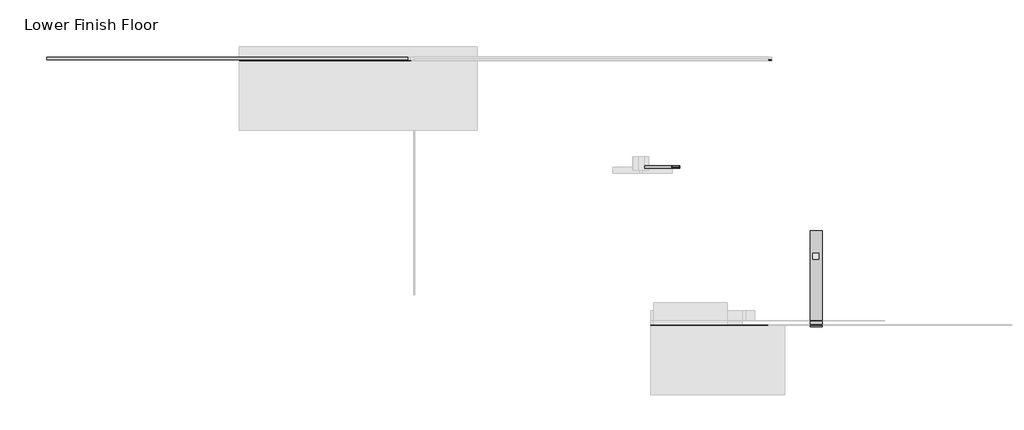
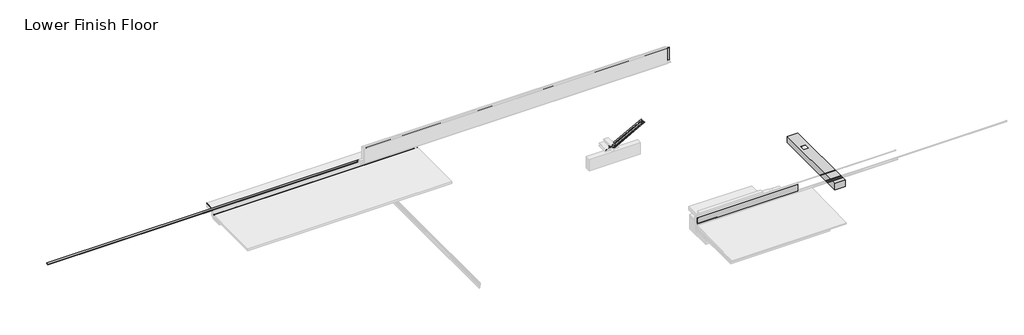
# One storey, part 1 of 2: 8 proxies, 2 beams.
"""IFC4 building model written with IfcOpenShell, lengths in millimetres."""

import ifcopenshell
import ifcopenshell.guid

model = None  # the IFC model being written
_history = None  # IfcOwnerHistory: only IFC2X3 demands one
_inside = {}  # id of a spatial element -> (the spatial element, [elements in it])
_under = {}  # id of a project, library or spatial element -> (it, [spatial elements below it])
_declared = {}  # id of a project -> (the project, [libraries it declares])
_typed = {}  # id of a type object -> (the type object, [elements of that type])
_made_of = {}  # id of a material, layer set ... -> (it, [elements and type objects made of it])


def new_model(schema):
    """Start an empty IFC model of exactly this schema.

    Asked for "IFC4X3", IfcOpenShell would pick the latest addendum, in which some entities
    have other attributes; the version numbers below select the first issue.
    IFC2X3 requires an IfcOwnerHistory on every rooted entity: one is made here for all.
    """
    global model, _history
    if schema == "IFC4X3":
        model = ifcopenshell.file(schema_version=(4, 3, 0, 0))
    else:
        model = ifcopenshell.file(schema=schema)
    _inside.clear()
    _under.clear()
    _declared.clear()
    _typed.clear()
    _made_of.clear()
    _history = None
    if model.schema == "IFC2X3":
        org = make("IfcOrganization", Name="unknown")
        user = make(
            "IfcPersonAndOrganization",
            ThePerson=make("IfcPerson", FamilyName="unknown"),
            TheOrganization=org,
        )
        app = make(
            "IfcApplication",
            ApplicationDeveloper=org,
            Version="unknown",
            ApplicationFullName="unknown",
            ApplicationIdentifier="unknown",
        )
        _history = make(
            "IfcOwnerHistory",
            OwningUser=user,
            OwningApplication=app,
            ChangeAction="ADDED",
            CreationDate=0,
        )
    return model


def make(cls, **values):
    """One entity of the class cls with the attributes given. An attribute that is None is left unset."""
    return model.create_entity(
        cls, **{name: value for name, value in values.items() if value is not None}
    )


def rooted(cls, **values):
    """An entity with a GlobalId (a new one), such as an element, a storey or a relation."""
    return make(cls, GlobalId=ifcopenshell.guid.new(), OwnerHistory=_history, **values)


def si_unit(unit_type, name, prefix=None):
    """IfcSIUnit, for example si_unit("LENGTHUNIT", "METRE", prefix="MILLI")."""
    return make("IfcSIUnit", UnitType=unit_type, Prefix=prefix, Name=name)


def assignment(units):
    """IfcUnitAssignment: the units of a project."""
    return None if units is None else make("IfcUnitAssignment", Units=units)


def point(xyz):
    """IfcCartesianPoint."""
    return None if xyz is None else make("IfcCartesianPoint", Coordinates=xyz)


def direction(xyz):
    """IfcDirection."""
    return None if xyz is None else make("IfcDirection", DirectionRatios=xyz)


def frame(location, z_axis=None, x_axis=None):
    """IfcAxis2Placement3D, a coordinate frame: its origin and axes. An axis left out is left unset."""
    return make(
        "IfcAxis2Placement3D",
        Location=point(location),
        Axis=direction(z_axis),
        RefDirection=direction(x_axis),
    )


def frame_2d(location, x_axis=None):
    """IfcAxis2Placement2D, a coordinate frame in the plane: its origin and x axis."""
    return make(
        "IfcAxis2Placement2D", Location=point(location), RefDirection=direction(x_axis)
    )


def origin():
    """The frame at (0, 0, 0) with its axes left unset."""
    return frame((0.0, 0.0, 0.0))


def place(relative_to, where):
    """IfcLocalPlacement: puts the frame where relative to a parent placement (None: the world)."""
    return make(
        "IfcLocalPlacement", PlacementRelTo=relative_to, RelativePlacement=where
    )


def context(
    kind, dimensions, precision=None, world=None, true_north=None, identifier=None
):
    """IfcGeometricRepresentationContext, for example the 3D "Model" context."""
    return make(
        "IfcGeometricRepresentationContext",
        ContextIdentifier=identifier,
        ContextType=kind,
        CoordinateSpaceDimension=dimensions,
        Precision=precision,
        WorldCoordinateSystem=world,
        TrueNorth=true_north,
    )


def project(units=None, contexts=None):
    """IfcProject with its units and contexts."""
    return rooted(
        "IfcProject",
        Name="project",
        RepresentationContexts=contexts,
        UnitsInContext=assignment(units),
    )


def spatial(cls, under=None, at=None, **own):
    """A site, building, storey or space (cls), placed at a placement, below another one or the project."""
    s = rooted(cls, ObjectPlacement=at, **own)
    if under is not None:
        _under.setdefault(under.id(), (under, []))[1].append(s)
    return s


def polyline(points):
    """IfcPolyline through the points."""
    return make("IfcPolyline", Points=[point(p) for p in points])


def circle_curve(where, radius):
    """IfcCircle in the frame where."""
    return make("IfcCircle", Position=where, Radius=radius)


def ellipse_curve(where, semi_axis1, semi_axis2):
    """IfcEllipse in the frame where."""
    return make(
        "IfcEllipse", Position=where, SemiAxis1=semi_axis1, SemiAxis2=semi_axis2
    )


def trimmed(basis, trim1, trim2, sense, master):
    """IfcTrimmedCurve: the piece of a basis curve between two trims."""
    return make(
        "IfcTrimmedCurve",
        BasisCurve=basis,
        Trim1=trim1,
        Trim2=trim2,
        SenseAgreement=sense,
        MasterRepresentation=master,
    )


def segment(curve, same_sense, transition):
    """IfcCompositeCurveSegment."""
    return make(
        "IfcCompositeCurveSegment",
        Transition=transition,
        SameSense=same_sense,
        ParentCurve=curve,
    )


def composite_curve(segments, self_intersect=None):
    """IfcCompositeCurve: segments joined end to end."""
    return make("IfcCompositeCurve", Segments=segments, SelfIntersect=self_intersect)


def outline(outer, holes=None, kind="AREA"):
    """IfcArbitraryClosedProfileDef: a profile drawn as a closed curve; with holes, ...WithVoids."""
    if holes is None:
        return make("IfcArbitraryClosedProfileDef", ProfileType=kind, OuterCurve=outer)
    return make(
        "IfcArbitraryProfileDefWithVoids",
        ProfileType=kind,
        OuterCurve=outer,
        InnerCurves=holes,
    )


def extrude(swept, where, along, depth):
    """IfcExtrudedAreaSolid: the profile swept, set in the frame where, extruded along a direction by depth."""
    return make(
        "IfcExtrudedAreaSolid",
        SweptArea=swept,
        Position=where,
        ExtrudedDirection=direction(along),
        Depth=depth,
    )


def shape(context_of_items, identifier, shape_type, items):
    """IfcShapeRepresentation: the items that make up one representation, for example the "Body"."""
    return make(
        "IfcShapeRepresentation",
        ContextOfItems=context_of_items,
        RepresentationIdentifier=identifier,
        RepresentationType=shape_type,
        Items=items,
    )


def source(mapping_origin, context_of_items, identifier, shape_type, items):
    """IfcRepresentationMap: a shape defined once, which mapped items show again and again."""
    return make(
        "IfcRepresentationMap",
        MappingOrigin=mapping_origin,
        MappedRepresentation=shape(context_of_items, identifier, shape_type, items),
    )


def transform(
    local_origin,
    x_axis=None,
    y_axis=None,
    z_axis=None,
    scale=None,
    scale2=None,
    scale3=None,
    uniform=True,
):
    """IfcCartesianTransformationOperator3D, or its non-uniform kind. x_axis, y_axis, z_axis: its Axis1, 2, 3."""
    if uniform:
        return make(
            "IfcCartesianTransformationOperator3D",
            Axis1=direction(x_axis),
            Axis2=direction(y_axis),
            LocalOrigin=point(local_origin),
            Scale=scale,
            Axis3=direction(z_axis),
        )
    return make(
        "IfcCartesianTransformationOperator3DnonUniform",
        Axis1=direction(x_axis),
        Axis2=direction(y_axis),
        LocalOrigin=point(local_origin),
        Scale=scale,
        Axis3=direction(z_axis),
        Scale2=scale2,
        Scale3=scale3,
    )


def mapped(mapping_source, mapping_target):
    """IfcMappedItem: shows the shape of a source again, moved by a transform."""
    return make(
        "IfcMappedItem", MappingSource=mapping_source, MappingTarget=mapping_target
    )


def made_of(thing, what):
    """Note that an element or type object is made of a material, layer set ...; save() writes the relation."""
    if what is not None:
        _made_of.setdefault(what.id(), (what, []))[1].append(thing)
    return thing


def element(
    cls,
    number,
    at=None,
    inside=None,
    cuts=None,
    type_object=None,
    material=None,
    context=None,
    identifier="Body",
    shape_type=None,
    held_by="IfcProductDefinitionShape",
    body=None,
    shapes=None,
    **own,
):
    """One element of the class cls, such as IfcWall. Its Tag is "e" and its number.

    at: its placement. inside: the storey or other place that contains it. cuts: it is an
    opening in that element (IfcRelVoidsElement). A single representation is given by context,
    identifier, shape_type and body (its items); several are given by shapes. held_by: the class
    of the entity that holds the representations. save() writes the other relations.
    """
    e = rooted(cls, Tag="e%d" % number, ObjectPlacement=at, **own)
    if body is not None:
        shapes = [shape(context, identifier, shape_type, body)]
    if shapes is not None:
        e.Representation = make(held_by, Representations=shapes)
    if inside is not None:
        _inside.setdefault(inside.id(), (inside, []))[1].append(e)
    if cuts is not None:
        rooted(
            "IfcRelVoidsElement", RelatingBuildingElement=cuts, RelatedOpeningElement=e
        )
    if type_object is not None:
        _typed.setdefault(type_object.id(), (type_object, []))[1].append(e)
    return made_of(e, material)


def aggregate(whole, parts):
    """IfcRelAggregates: a whole, such as a stair, and the parts it consists of."""
    return rooted("IfcRelAggregates", RelatingObject=whole, RelatedObjects=parts)


def save(model, path):
    """Write the relations noted so far, then the file.

    IfcRelAggregates (storeys below a building ...), IfcRelContainedInSpatialStructure (elements
    in a storey), IfcRelDefinesByType, IfcRelAssociatesMaterial and IfcRelDeclares: one each for
    every whole, place, type object, material and project.
    """
    for whole, parts in _under.values():
        aggregate(whole, parts)
    for where, things in _inside.values():
        rooted(
            "IfcRelContainedInSpatialStructure",
            RelatedElements=things,
            RelatingStructure=where,
        )
    for kind, things in _typed.values():
        rooted("IfcRelDefinesByType", RelatedObjects=things, RelatingType=kind)
    for what, things in _made_of.values():
        rooted("IfcRelAssociatesMaterial", RelatedObjects=things, RelatingMaterial=what)
    for by, libraries in _declared.values():
        rooted("IfcRelDeclares", RelatingContext=by, RelatedDefinitions=libraries)
    model.write(path)


def plane_surface(at):
    """IfcPlane: the flat surface through the origin of the frame at, square to its z axis."""
    return make("IfcPlane", Position=at)


def cylinder_surface(at, radius):
    """IfcCylindricalSurface: all points at the distance radius from the z axis of the frame at."""
    return make("IfcCylindricalSurface", Position=at, Radius=radius)


def revolved_surface(curve, axis_point, axis_direction):
    """IfcSurfaceOfRevolution: the curve turned about the line through axis_point along axis_direction."""
    return make(
        "IfcSurfaceOfRevolution",
        SweptCurve=make("IfcArbitraryOpenProfileDef", ProfileType="CURVE", Curve=curve),
        AxisPosition=make("IfcAxis1Placement", Location=point(axis_point), Axis=direction(axis_direction)),
    )


def advanced_brep(points, edges, surfaces, faces):
    """IfcAdvancedBrep: a solid bounded by faces that lie on surfaces and meet in shared edges.

    An edge is (start, end): straight between two places in points (the first is 0);
    or (start, end, curve); or (start, end, curve, False) where it runs against its curve.
    A face is (place in surfaces, loops), or (place, loops, False) where it looks against
    its surface's normal. A loop lists edges by number (the first is 1), with a minus sign
    where the edge is run from its end to its start. The first loop is the outer one.
    """
    corners = [point(p) for p in points]
    vertices = [make("IfcVertexPoint", VertexGeometry=c) for c in corners]
    made = []
    for start, end, *more in edges:
        made.append(
            make(
                "IfcEdgeCurve",
                EdgeStart=vertices[start],
                EdgeEnd=vertices[end],
                EdgeGeometry=more[0] if more else make("IfcPolyline", Points=[corners[start], corners[end]]),
                SameSense=more[1] if len(more) > 1 else True,
            )
        )
    hull = []
    for where, loops, *sense in faces:
        bounds = []
        for j, loop in enumerate(loops):
            ring = [make("IfcOrientedEdge", EdgeElement=made[abs(k) - 1], Orientation=k > 0) for k in loop]
            bounds.append(
                make(
                    "IfcFaceOuterBound" if j == 0 else "IfcFaceBound",
                    Bound=make("IfcEdgeLoop", EdgeList=ring),
                    Orientation=True,
                )
            )
        hull.append(make("IfcAdvancedFace", Bounds=bounds, FaceSurface=surfaces[where], SameSense=sense[0] if sense else True))
    return make("IfcAdvancedBrep", Outer=make("IfcClosedShell", CfsFaces=hull))


def w_wide_flange_w10x22_c2580360(model_context):
    return source(origin(), model_context, "Body", "SweptSolid", [
        extrude(outline(composite_curve([segment(polyline([(73.025, -120.396), (73.025, -129.54), (-73.025, -129.54), (-73.025, -120.396), (-17.7165, -120.396)]), True, "CONTINUOUS"), segment(trimmed(circle_curve(frame_2d((-17.7165, -105.7275)), 14.6685), [point((-17.7165, -120.396))], [point((-3.048, -105.7275))], True, "CARTESIAN"), True, "CONTINUOUS"), segment(polyline([(-3.048, -105.7275), (-3.048, 105.7275)]), True, "CONTINUOUS"), segment(trimmed(circle_curve(frame_2d((-17.7165, 105.7275)), 14.6685), [point((-3.048, 105.7275))], [point((-17.7165, 120.396))], True, "CARTESIAN"), True, "CONTINUOUS"), segment(polyline([(-17.7165, 120.396), (-73.025, 120.396), (-73.025, 129.54), (73.025, 129.54), (73.025, 120.396), (17.7165, 120.396)]), True, "CONTINUOUS"), segment(trimmed(circle_curve(frame_2d((17.7165, 105.7275)), 14.6685), [point((17.7165, 120.396))], [point((3.048, 105.7275))], True, "CARTESIAN"), True, "CONTINUOUS"), segment(polyline([(3.048, 105.7275), (3.048, -105.7275)]), True, "CONTINUOUS"), segment(trimmed(circle_curve(frame_2d((17.7165, -105.7275)), 14.6685), [point((3.048, -105.7275))], [point((17.7165, -120.396))], True, "CARTESIAN"), True, "CONTINUOUS"), segment(polyline([(17.7165, -120.396), (73.025, -120.396)]), True, "CONTINUOUS")], self_intersect=False)), frame((-558.8, 0.0, 0.0), z_axis=(1.0, 0.0, 0.0), x_axis=(0.0, 1.0, 0.0)), (0.0, 0.0, 1.0), 1117.6),
    ])


def generic_models_109_generic_models_1_7cfb6ed3(model_context):
    return source(origin(), model_context, "Body", "SweptSolid", [
        extrude(outline(polyline([(-20998.9733045, 51294.7476718), (-20998.9733045, 51434.4476718), (-1948.9733045, 51434.4476718), (-1948.9733045, 51294.7476718), (-20998.9733045, 51294.7476718)])), frame((0.0, 0.0, 127066.3735933), z_axis=(0.0, 0.0, 1.0), x_axis=(1.0, 0.0, 0.0)), (0.0, 0.0, 1.0), 38.1),
    ])


def generic_models_141_generic_models_4_645eafa7(model_context):
    return source(origin(), model_context, "Body", "SweptSolid", [
        extrude(outline(polyline([(-2152.1733045, 51452.647716), (-2152.1733045, 51433.597716), (-20795.7733045, 51433.597716), (-20795.7733045, 51452.647716), (-2152.1733045, 51452.647716)])), frame((0.0, 0.0, 126384.0358061), z_axis=(0.0, 0.0, 1.0), x_axis=(1.0, 0.0, 0.0)), (0.0, 0.0, 1.0), 780.3940166),
    ])


def generic_models_142_generic_models_4_bf06cd15(model_context):
    return source(origin(), model_context, "Body", "SweptSolid", [
        extrude(outline(polyline([(20644.6159513, 7056.3254549), (20644.6159513, 7069.0254549), (33192.2159513, 7069.0254549), (33192.2159513, 7056.3254549), (20644.6159513, 7056.3254549)])), frame((0.0, 0.0, 123786.1261094), z_axis=(0.0, 0.0, 1.0), x_axis=(1.0, 0.0, 0.0)), (0.0, 0.0, 1.0), 114.3112934),
    ])


def generic_models_144_generic_models_4_d644e738(model_context):
    return source(origin(), model_context, "Body", "SweptSolid", [
        extrude(outline(polyline([(20644.6159513, 7212.6867903), (20644.6159513, 7761.1754549), (33192.2159513, 7761.1754549), (33192.2159513, 7212.6867903), (20644.6159513, 7212.6867903)])), frame((0.0, 0.0, 124030.3826265), z_axis=(0.0, 0.0, 1.0), x_axis=(1.0, 0.0, 0.0)), (0.0, 0.0, 1.0), 17.4625),
    ])


def generic_models_146_generic_models_4_285cb4c9(model_context):
    return source(origin(), model_context, "Body", "SweptSolid", [
        extrude(outline(polyline([(20644.6159513, 7212.6867903), (20644.6159513, 7761.1754549), (33192.2159513, 7761.1754549), (33192.2159513, 7212.6867903), (20644.6159513, 7212.6867903)])), frame((0.0, 0.0, 124028.7951265), z_axis=(0.0, 0.0, 1.0), x_axis=(1.0, 0.0, 0.0)), (0.0, 0.0, 1.0), 1.5875),
    ])


def generic_models_148_generic_models_1_1e1312a9(model_context):
    return source(origin(), model_context, "Body", "SweptSolid", [
        extrude(outline(composite_curve([segment(trimmed(circle_curve(frame_2d((7062.6754549, 123920.3246075)), 8.620055), [point((7056.3254549, 123914.4951265))], [point((7069.0254549, 123914.4951265))], True, "CARTESIAN"), True, "CONTINUOUS"), segment(polyline([(7069.0254549, 123914.4951265), (7069.0254549, 123904.9701265)]), True, "CONTINUOUS"), segment(trimmed(circle_curve(frame_2d((7062.6754549, 123910.7996075)), 8.620055), [point((7069.0254549, 123904.9701265))], [point((7056.3254549, 123904.9701265))], False, "CARTESIAN"), True, "CONTINUOUS"), segment(polyline([(7056.3254549, 123904.9701265), (7056.3254549, 123914.4951265)]), True, "CONTINUOUS")], self_intersect=False)), frame((20644.6159513, 0.0, 0.0), z_axis=(1.0, 0.0, 0.0), x_axis=(0.0, 1.0, 0.0)), (0.0, 0.0, 1.0), 12344.4),
    ])


model = new_model("IFC4")

# Units and contexts
model_context = context("Model", 3, world=origin())
ifc_project = project(units=[si_unit("LENGTHUNIT", "METRE", prefix="MILLI")], contexts=[model_context])

# Site, building, storey
site = spatial("IfcSite", under=ifc_project)
building = spatial("IfcBuilding", under=site)
storey = spatial("IfcBuildingStorey", under=building, Name="Lower Finish Floor", Elevation=123297.696)

# Beams
placement = place(None, origin())
w_wide_flange_w10x22_shape = w_wide_flange_w10x22_c2580360(model_context)
element("IfcBeam", 1, ObjectType="W-Wide Flange : W10X22", at=placement, inside=storey, context=model_context, shape_type="MappedRepresentation", body=[
    mapped(w_wide_flange_w10x22_shape, transform((4044.9556307, -6661.7592785, 123168.156), x_axis=(1.0, 0.0, 0.0), y_axis=(0.0, 1.0, 0.0), z_axis=(0.0, 0.0, 1.0))),
])
element("IfcBeam", 2, ObjectType="W-Wide Flange1 : W8X21  stairs bottom", at=placement, inside=storey, context=model_context, shape_type="AdvancedBrep", body=[
    advanced_brep(
    [(1470.7410726, 1304.8540131, 123264.3525795), (1475.5851696, 1304.8540131, 123255.4668916), (1475.5851696, 1171.0079193, 123255.4668916), (1470.7410726, 1171.0079193, 123264.3525795), (1470.7410726, 1214.7137787, 123264.3525795), (1461.1478608, 1234.7559662, 123281.949726), (1389.3412457, 1234.7559662, 123413.6669814), (1379.7480339, 1214.7137787, 123431.264128), (1379.7480339, 1171.0079193, 123431.264128), (1374.9039368, 1171.0079193, 123440.1498159), (1374.9039368, 1304.8540131, 123440.1498159), (1379.7480339, 1304.8540131, 123431.264128), (1379.7480339, 1261.1481537, 123431.264128), (1389.3412457, 1241.1059662, 123413.6669814), (1461.1478608, 1241.1059662, 123281.949726), (1470.7410726, 1261.1481537, 123264.3525795), (3712.011804, 1261.1481537, 124486.1975398), (3712.011804, 1304.8540131, 124486.1975398), (3670.1395627, 1241.1059662, 124486.1975398), (3601.1574357, 1241.1059662, 124619.4545853), (3601.1574357, 1241.1059662, 124510.0100398), (3586.4889357, 1241.1059662, 124495.3415398), (3531.1804357, 1241.1059662, 124495.3415398), (3531.1804357, 1241.1059662, 124486.1975398), (3601.1574357, 1261.1481537, 124642.2815407), (3601.1574357, 1304.8540131, 124642.2815407), (3601.1574357, 1304.8540131, 124653.8080231), (3601.1574357, 1171.0079193, 124653.8080231), (3601.1574357, 1171.0079193, 124642.2815407), (3601.1574357, 1214.7137787, 124642.2815407), (3601.1574357, 1234.7559662, 124619.4545853), (3670.1395627, 1234.7559662, 124486.1975398), (3531.1804357, 1234.7559662, 124486.1975398), (3531.1804357, 1234.7559662, 124495.3415398), (3586.4889357, 1234.7559662, 124495.3415398), (3601.1574357, 1234.7559662, 124510.0100398), (3712.011804, 1214.7137787, 124486.1975398), (3712.011804, 1171.0079193, 124486.1975398), (3733.155213, 1171.0079193, 124486.1975398), (3733.155213, 1304.8540131, 124486.1975398)],
    [
        (0, 1),
        (1, 2),
        (2, 3),
        (3, 4),
        (4, 5, circle_curve(frame((1461.1478608, 1214.7137787, 123281.949726), z_axis=(0.8780052855906307, 0.0, 0.47865093593861807), x_axis=(0.0, -1.0, 0.0)), 20.0421875)),
        (5, 6),
        (6, 7, circle_curve(frame((1389.3412457, 1214.7137787, 123413.6669814), z_axis=(0.8780052855906307, 0.0, 0.47865093593861807), x_axis=(0.0, -1.0, 0.0)), 20.0421875)),
        (7, 8),
        (8, 9),
        (9, 10),
        (10, 11),
        (11, 12),
        (12, 13, circle_curve(frame((1389.3412457, 1261.1481537, 123413.6669814), z_axis=(0.8780052855906307, 0.0, 0.47865093593861807), x_axis=(0.0, -1.0, 0.0)), 20.0421875)),
        (13, 14),
        (14, 15, circle_curve(frame((1461.1478608, 1261.1481537, 123281.949726), z_axis=(0.8780052855906307, 0.0, 0.47865093593861807), x_axis=(0.0, -1.0, 0.0)), 20.0421875)),
        (15, 0),
        (15, 16),
        (16, 17),
        (17, 0),
        (14, 18),
        (18, 16, ellipse_curve(frame((3670.1395627, 1261.1481537, 124486.1975398), z_axis=(0.0, 0.0, 1.0), x_axis=(-1.0, 0.0, 0.0)), 41.8722413, 20.0421875)),
        (13, 19),
        (19, 20),
        (20, 21, circle_curve(frame((3586.4889357, 1241.1059662, 124510.0100398), z_axis=(0.0, 1.0, 0.0), x_axis=(0.8780052855906307, 0.0, 0.47865093593861807)), 14.6685)),
        (21, 22),
        (22, 23),
        (23, 18),
        (12, 24),
        (24, 19, ellipse_curve(frame((3601.1574357, 1261.1481537, 124619.4545853), z_axis=(1.0, 0.0, 0.0), x_axis=(0.0, 0.0, -1.0)), 22.8269554, 20.0421875)),
        (11, 25),
        (25, 24),
        (10, 26),
        (26, 25),
        (9, 27),
        (27, 26),
        (8, 28),
        (28, 27),
        (7, 29),
        (29, 28),
        (6, 30),
        (30, 29, ellipse_curve(frame((3601.1574357, 1214.7137787, 124619.4545853), z_axis=(1.0, 0.0, 0.0), x_axis=(0.0, 0.0, -1.0)), 22.8269554, 20.0421875)),
        (5, 31),
        (31, 32),
        (32, 33),
        (33, 34),
        (34, 35, circle_curve(frame((3586.4889357, 1234.7559662, 124510.0100398), z_axis=(0.0, -1.0, 0.0), x_axis=(0.8780052855906307, 0.0, 0.47865093593861807)), 14.6685)),
        (35, 30),
        (4, 36),
        (36, 31, ellipse_curve(frame((3670.1395627, 1214.7137787, 124486.1975398), z_axis=(0.0, 0.0, 1.0), x_axis=(-1.0, 0.0, 0.0)), 41.8722413, 20.0421875)),
        (3, 37),
        (37, 36),
        (2, 38),
        (38, 37),
        (1, 39),
        (39, 38),
        (17, 39),
        (32, 23),
        (22, 33),
        (21, 34),
        (20, 35),
    ],
    [
        plane_surface(frame((1425.2445532, 1237.9309662, 123347.8083537), z_axis=(-0.8780052855906311, 0.0, -0.47865093593861746), x_axis=(-0.47865093593861746, 0.0, 0.8780052855906311))),
        plane_surface(frame((3866.2039334, 1304.8540131, 124570.256495), z_axis=(-0.47865093593861807, 0.0, 0.8780052855906307), x_axis=(-0.8780052855906307, 0.0, -0.47865093593861807))),
        revolved_surface(polyline([(1461.147860779813, 1241.1059662, 123281.94972603704), (3702.4185922197667, 1241.1059662, 124503.79468631413)]), (3856.6107216, 1261.1481537, 124587.8536416), (-0.8780052855906307, 0.0, -0.47865093593861807)),
        plane_surface(frame((3856.6107216, 1241.1059662, 124587.8536416), z_axis=(0.0, 1.0, 0.0), x_axis=(-0.8780052855906307, 0.0, -0.47865093593861807))),
        revolved_surface(polyline([(1389.3412456798133, 1241.1059662, 123413.66698143704), (3610.750647509506, 1241.1059662, 124624.68439413219)]), (3784.8041065, 1261.1481537, 124719.570897), (-0.8780052855906307, 0.0, -0.47865093593861807)),
        plane_surface(frame((3775.2108947, 1261.1481537, 124737.1680436), z_axis=(0.47865093593861807, 0.0, -0.8780052855906307), x_axis=(-0.8780052855906307, 0.0, -0.47865093593861807))),
        plane_surface(frame((3775.2108947, 1304.8540131, 124737.1680436), z_axis=(0.0, 1.0, 0.0), x_axis=(-0.8780052855906307, 0.0, -0.47865093593861807))),
        plane_surface(frame((3770.3667976, 1304.8540131, 124746.0537314), z_axis=(-0.47865093593861807, 0.0, 0.8780052855906307), x_axis=(-0.8780052855906307, 0.0, -0.47865093593861807))),
        plane_surface(frame((3770.3667976, 1171.0079193, 124746.0537314), z_axis=(0.0, -1.0, 0.0), x_axis=(-0.8780052855906307, 0.0, -0.47865093593861807))),
        plane_surface(frame((3775.2108947, 1171.0079193, 124737.1680436), z_axis=(0.47865093593861807, 0.0, -0.8780052855906307), x_axis=(-0.8780052855906307, 0.0, -0.47865093593861807))),
        revolved_surface(polyline([(1389.3412456798133, 1194.6715912, 123413.66698143704), (3610.750647509506, 1194.6715912, 124624.68439413219)]), (3784.8041065, 1214.7137787, 124719.570897), (-0.8780052855906307, 0.0, -0.47865093593861807)),
        plane_surface(frame((3784.8041065, 1234.7559662, 124719.570897), z_axis=(0.0, -1.0, 0.0), x_axis=(-0.8780052855906307, 0.0, -0.47865093593861807))),
        revolved_surface(polyline([(1461.147860779813, 1194.6715912, 123281.94972603704), (3702.4185922197667, 1194.6715912, 124503.79468631413)]), (3856.6107216, 1214.7137787, 124587.8536416), (-0.8780052855906307, 0.0, -0.47865093593861807)),
        plane_surface(frame((3866.2039334, 1214.7137787, 124570.256495), z_axis=(-0.47865093593861807, 0.0, 0.8780052855906307), x_axis=(-0.8780052855906307, 0.0, -0.47865093593861807))),
        plane_surface(frame((3866.2039334, 1171.0079193, 124570.256495), z_axis=(0.0, -1.0, 0.0), x_axis=(-0.8780052855906307, 0.0, -0.47865093593861807))),
        plane_surface(frame((3871.0480304, 1171.0079193, 124561.3708072), z_axis=(0.47865093593861807, 0.0, -0.8780052855906307), x_axis=(-0.8780052855906307, 0.0, -0.47865093593861807))),
        plane_surface(frame((3871.0480304, 1304.8540131, 124561.3708072), z_axis=(0.0, 1.0, 0.0), x_axis=(-0.8780052855906307, 0.0, -0.47865093593861807))),
        plane_surface(frame((3531.1804357, 4006.5309662, 124486.1975398), z_axis=(1.0, 0.0, 0.0), x_axis=(0.0, -1.0, 0.0))),
        plane_surface(frame((3531.1804357, 4006.5309662, 124495.3415398), z_axis=(0.0, 0.0, -1.0), x_axis=(0.0, -1.0, 0.0))),
        cylinder_surface(frame((3586.4889357, -1530.6690338, 124510.0100398), z_axis=(0.0, -1.0, 0.0), x_axis=(0.8780052855906307, 0.0, 0.47865093593861807)), 14.6685),
        plane_surface(frame((3601.1574357, 4006.5309662, 124510.0100398), z_axis=(1.0, 0.0, 0.0), x_axis=(0.0, -1.0, 0.0))),
        plane_surface(frame((4020.1506251, 4006.5309662, 124486.1975398), z_axis=(0.0, 0.0, 1.0), x_axis=(0.0, -1.0, 0.0))),
    ],
    [
        (0, [[1, 2, 3, 4, 5, 6, 7, 8, 9, 10, 11, 12, 13, 14, 15, 16]]),
        (1, [[-16, 17, 18, 19]]),
        (2, [[-15, 20, 21, -17]]),
        (3, [[-14, 22, 23, 24, 25, 26, 27, -20]]),
        (4, [[-13, 28, 29, -22]]),
        (5, [[-12, 30, 31, -28]]),
        (6, [[-11, 32, 33, -30]]),
        (7, [[-10, 34, 35, -32]]),
        (8, [[-9, 36, 37, -34]]),
        (9, [[-8, 38, 39, -36]]),
        (10, [[-7, 40, 41, -38]]),
        (11, [[-6, 42, 43, 44, 45, 46, 47, -40]]),
        (12, [[-5, 48, 49, -42]]),
        (13, [[-4, 50, 51, -48]]),
        (14, [[-3, 52, 53, -50]]),
        (15, [[-2, 54, 55, -52]]),
        (16, [[-1, -19, 56, -54]]),
        (17, [[57, -26, 58, -44]]),
        (18, [[-58, -25, 59, -45]]),
        (19, [[-59, -24, 60, -46]]),
        (20, [[-60, -23, -29, -31, -33, -35, -37, -39, -41, -47]]),
        (21, [[-57, -43, -49, -51, -53, -55, -56, -18, -21, -27]]),
    ],
),
    advanced_brep(
    [(1811.4563888, 1261.1481537, 123450.096), (1811.4563888, 1304.8540131, 123450.096), (1832.5997978, 1304.8540131, 123450.096), (1832.5997978, 1171.0079193, 123450.096), (1811.4563888, 1171.0079193, 123450.096), (1811.4563888, 1214.7137787, 123450.096), (1769.5841475, 1234.7559662, 123450.096), (1456.1642025, 1234.7559662, 123450.096), (1414.2919612, 1214.7137787, 123450.096), (1414.2919612, 1171.0079193, 123450.096), (1393.1485522, 1171.0079193, 123450.096), (1393.1485522, 1304.8540131, 123450.096), (1414.2919612, 1304.8540131, 123450.096), (1414.2919612, 1261.1481537, 123450.096), (1456.1642025, 1241.1059662, 123450.096), (1769.5841475, 1241.1059662, 123450.096), (3670.1395627, 1241.1059662, 124486.1975398), (3712.011804, 1261.1481537, 124486.1975398), (3712.011804, 1304.8540131, 124486.1975398), (3531.1804357, 1241.1059662, 124486.1975398), (3531.1804357, 1234.7559662, 124486.1975398), (3670.1395627, 1234.7559662, 124486.1975398), (3712.011804, 1214.7137787, 124486.1975398), (3712.011804, 1171.0079193, 124486.1975398), (3733.155213, 1171.0079193, 124486.1975398), (3733.155213, 1304.8540131, 124486.1975398), (3601.1574357, 1241.1059662, 124619.4545853), (3601.1574357, 1241.1059662, 124510.0100398), (3586.4889357, 1241.1059662, 124495.3415398), (3531.1804357, 1241.1059662, 124495.3415398), (3601.1574357, 1261.1481537, 124642.2815407), (3601.1574357, 1234.7559662, 124510.0100398), (3601.1574357, 1304.8540131, 124642.2815407), (3601.1574357, 1304.8540131, 124653.8080231), (3601.1574357, 1171.0079193, 124653.8080231), (3601.1574357, 1171.0079193, 124642.2815407), (3601.1574357, 1214.7137787, 124642.2815407), (3601.1574357, 1234.7559662, 124619.4545853), (3586.4889357, 1234.7559662, 124495.3415398), (3531.1804357, 1234.7559662, 124495.3415398)],
    [
        (0, 1),
        (1, 2),
        (2, 3),
        (3, 4),
        (4, 5),
        (5, 6, ellipse_curve(frame((1769.5841475, 1214.7137787, 123450.096), z_axis=(0.0, 0.0, 1.0), x_axis=(-1.0, 0.0, 0.0)), 41.8722413, 20.0421875)),
        (6, 7),
        (7, 8, ellipse_curve(frame((1456.1642025, 1214.7137787, 123450.096), z_axis=(0.0, 0.0, 1.0), x_axis=(-1.0, 0.0, 0.0)), 41.8722413, 20.0421875)),
        (8, 9),
        (9, 10),
        (10, 11),
        (11, 12),
        (12, 13),
        (13, 14, ellipse_curve(frame((1456.1642025, 1261.1481537, 123450.096), z_axis=(0.0, 0.0, 1.0), x_axis=(-1.0, 0.0, 0.0)), 41.8722413, 20.0421875)),
        (14, 15),
        (15, 0, ellipse_curve(frame((1769.5841475, 1261.1481537, 123450.096), z_axis=(0.0, 0.0, 1.0), x_axis=(-1.0, 0.0, 0.0)), 41.8722413, 20.0421875)),
        (15, 16),
        (16, 17, ellipse_curve(frame((3670.1395627, 1261.1481537, 124486.1975398), z_axis=(0.0, 0.0, 1.0), x_axis=(-1.0, 0.0, 0.0)), 41.8722413, 20.0421875)),
        (17, 0),
        (17, 18),
        (18, 1),
        (19, 20),
        (20, 21),
        (21, 22, ellipse_curve(frame((3670.1395627, 1214.7137787, 124486.1975398), z_axis=(0.0, 0.0, -1.0), x_axis=(-1.0, 0.0, 0.0)), 41.8722413, 20.0421875)),
        (22, 23),
        (23, 24),
        (24, 25),
        (25, 18),
        (16, 19),
        (25, 2),
        (14, 26),
        (26, 27),
        (27, 28, circle_curve(frame((3586.4889357, 1241.1059662, 124510.0100398), z_axis=(0.0, 1.0, 0.0), x_axis=(0.8780052855906307, 0.0, 0.47865093593861807)), 14.6685)),
        (28, 29),
        (29, 19),
        (13, 30),
        (30, 26, ellipse_curve(frame((3601.1574357, 1261.1481537, 124619.4545853), z_axis=(1.0, 0.0, 0.0), x_axis=(0.0, 0.0, -1.0)), 22.8269554, 20.0421875)),
        (31, 27),
        (30, 32),
        (32, 33),
        (33, 34),
        (34, 35),
        (35, 36),
        (36, 37, ellipse_curve(frame((3601.1574357, 1214.7137787, 124619.4545853), z_axis=(-1.0, 0.0, 0.0), x_axis=(0.0, 0.0, -1.0)), 22.8269554, 20.0421875)),
        (37, 31),
        (38, 28),
        (31, 38, circle_curve(frame((3586.4889357, 1234.7559662, 124510.0100398), z_axis=(0.0, 1.0, 0.0), x_axis=(0.8780052855906307, 0.0, 0.47865093593861807)), 14.6685)),
        (39, 29),
        (38, 39),
        (39, 20),
        (12, 32),
        (11, 33),
        (10, 34),
        (9, 35),
        (8, 36),
        (7, 37),
        (6, 21),
        (5, 22),
        (4, 23),
        (3, 24),
    ],
    [
        plane_surface(frame((1454.6447649, 1136.0769662, 123450.096), z_axis=(0.0, 0.0, -1.0), x_axis=(-1.0, 0.0, 0.0))),
        revolved_surface(polyline([(1737.305117987853, 1241.1059662, 123432.4988534719), (3702.4185922197667, 1241.1059662, 124503.79468631413)]), (3856.6107216, 1261.1481537, 124587.8536416), (-0.8780052855906307, 0.0, -0.47865093593861807)),
        plane_surface(frame((3866.2039334, 1304.8540131, 124570.256495), z_axis=(-0.47865093593861807, 0.0, 0.8780052855906307), x_axis=(-0.8780052855906307, 0.0, -0.47865093593861807))),
        plane_surface(frame((4020.1506251, 4006.5309662, 124486.1975398), z_axis=(0.0, 0.0, 1.0), x_axis=(0.0, -1.0, 0.0))),
        plane_surface(frame((3871.0480304, 1304.8540131, 124561.3708072), z_axis=(0.0, 1.0, 0.0), x_axis=(-0.8780052855906307, 0.0, -0.47865093593861807))),
        plane_surface(frame((3856.6107216, 1241.1059662, 124587.8536416), z_axis=(0.0, 1.0, 0.0), x_axis=(-0.8780052855906307, 0.0, -0.47865093593861807))),
        revolved_surface(polyline([(1423.8851730104411, 1241.1059662, 123432.49885343047), (3610.750647509506, 1241.1059662, 124624.68439413219)]), (3784.8041065, 1261.1481537, 124719.570897), (-0.8780052855906307, 0.0, -0.47865093593861807)),
        plane_surface(frame((3601.1574357, 4006.5309662, 124510.0100398), z_axis=(1.0, 0.0, 0.0), x_axis=(0.0, -1.0, 0.0))),
        cylinder_surface(frame((3586.4889357, -1530.6690338, 124510.0100398), z_axis=(0.0, -1.0, 0.0), x_axis=(0.8780052855906307, 0.0, 0.47865093593861807)), 14.6685),
        plane_surface(frame((3531.1804357, 4006.5309662, 124495.3415398), z_axis=(0.0, 0.0, -1.0), x_axis=(0.0, -1.0, 0.0))),
        plane_surface(frame((3531.1804357, 4006.5309662, 124486.1975398), z_axis=(1.0, 0.0, 0.0), x_axis=(0.0, -1.0, 0.0))),
        plane_surface(frame((3775.2108947, 1261.1481537, 124737.1680436), z_axis=(0.47865093593861807, 0.0, -0.8780052855906307), x_axis=(-0.8780052855906307, 0.0, -0.47865093593861807))),
        plane_surface(frame((3775.2108947, 1304.8540131, 124737.1680436), z_axis=(0.0, 1.0, 0.0), x_axis=(-0.8780052855906307, 0.0, -0.47865093593861807))),
        plane_surface(frame((3770.3667976, 1304.8540131, 124746.0537314), z_axis=(-0.47865093593861807, 0.0, 0.8780052855906307), x_axis=(-0.8780052855906307, 0.0, -0.47865093593861807))),
        plane_surface(frame((3770.3667976, 1171.0079193, 124746.0537314), z_axis=(0.0, -1.0, 0.0), x_axis=(-0.8780052855906307, 0.0, -0.47865093593861807))),
        plane_surface(frame((3775.2108947, 1171.0079193, 124737.1680436), z_axis=(0.47865093593861807, 0.0, -0.8780052855906307), x_axis=(-0.8780052855906307, 0.0, -0.47865093593861807))),
        revolved_surface(polyline([(1423.8851730104411, 1194.6715912, 123432.49885343047), (3610.750647509506, 1194.6715912, 124624.68439413219)]), (3784.8041065, 1214.7137787, 124719.570897), (-0.8780052855906307, 0.0, -0.47865093593861807)),
        plane_surface(frame((3784.8041065, 1234.7559662, 124719.570897), z_axis=(0.0, -1.0, 0.0), x_axis=(-0.8780052855906307, 0.0, -0.47865093593861807))),
        revolved_surface(polyline([(1737.305117987853, 1194.6715912, 123432.4988534719), (3702.4185922197667, 1194.6715912, 124503.79468631413)]), (3856.6107216, 1214.7137787, 124587.8536416), (-0.8780052855906307, 0.0, -0.47865093593861807)),
        plane_surface(frame((3866.2039334, 1214.7137787, 124570.256495), z_axis=(-0.47865093593861807, 0.0, 0.8780052855906307), x_axis=(-0.8780052855906307, 0.0, -0.47865093593861807))),
        plane_surface(frame((3866.2039334, 1171.0079193, 124570.256495), z_axis=(0.0, -1.0, 0.0), x_axis=(-0.8780052855906307, 0.0, -0.47865093593861807))),
        plane_surface(frame((3871.0480304, 1171.0079193, 124561.3708072), z_axis=(0.47865093593861807, 0.0, -0.8780052855906307), x_axis=(-0.8780052855906307, 0.0, -0.47865093593861807))),
    ],
    [
        (0, [[1, 2, 3, 4, 5, 6, 7, 8, 9, 10, 11, 12, 13, 14, 15, 16]]),
        (1, [[17, 18, 19, -16]]),
        (2, [[-19, 20, 21, -1]]),
        (3, [[22, 23, 24, 25, 26, 27, 28, -20, -18, 29]]),
        (4, [[-21, -28, 30, -2]]),
        (5, [[31, 32, 33, 34, 35, -29, -17, -15]]),
        (6, [[36, 37, -31, -14]]),
        (7, [[38, -32, -37, 39, 40, 41, 42, 43, 44, 45]]),
        (8, [[46, -33, -38, 47]]),
        (9, [[48, -34, -46, 49]]),
        (10, [[-22, -35, -48, 50]]),
        (11, [[51, -39, -36, -13]]),
        (12, [[52, -40, -51, -12]]),
        (13, [[53, -41, -52, -11]]),
        (14, [[54, -42, -53, -10]]),
        (15, [[55, -43, -54, -9]]),
        (16, [[56, -44, -55, -8]]),
        (17, [[57, -23, -50, -49, -47, -45, -56, -7]]),
        (18, [[58, -24, -57, -6]]),
        (19, [[59, -25, -58, -5]]),
        (20, [[60, -26, -59, -4]]),
        (21, [[-30, -27, -60, -3]]),
    ],
),
])

# Proxies
element("IfcBuildingElementProxy", 3, Name="Generic Models 116 : Generic Models 3", ObjectType="Generic Models 116 : Generic Models 3", at=placement, inside=storey, context=model_context, shape_type="AdvancedBrep", body=[
    advanced_brep(
    [(11250.1962575, -7185.1295431, 122737.5366172), (11250.1962575, -7185.1295431, 123145.296), (10606.836186, -7185.1295431, 123145.296), (10606.836186, -7185.1295431, 122737.5366172), (10606.836186, -2109.6309403, 123145.296), (11250.1962575, -2109.6309403, 123145.296), (11250.1962575, -2109.6309403, 122737.5366172), (10606.836186, -2109.6309403, 122737.5366172), (11050.9203062, -3603.6670282, 123145.296), (10758.8203062, -3603.6670282, 123145.296), (10758.8203062, -3298.8670282, 123145.296), (11050.9203062, -3298.8670282, 123145.296), (10795.3734607, -3298.8670282, 123132.596), (10801.7234607, -3292.5170282, 123132.596), (10808.0734607, -3298.8670282, 123132.596), (10801.7234607, -3292.5170282, 122878.596), (10801.7234607, -3305.2170282, 123132.596), (10801.7234607, -3305.2170282, 122878.596), (10883.7654841, -3305.2170282, 122878.596), (10883.7654841, -3292.5170282, 122878.596), (10998.5558717, -3298.8670282, 123132.596), (11004.9058717, -3292.5170282, 123132.596), (11011.2558717, -3298.8670282, 123132.596), (11004.9058717, -3305.2170282, 122878.596), (11004.9058717, -3305.2170282, 123132.596), (11004.9058717, -3292.5170282, 122878.596), (10922.8638483, -3305.2170282, 122878.596), (10922.8638483, -3292.5170282, 122878.596), (10758.8203062, -3603.6670282, 123132.596), (11050.9203062, -3603.6670282, 123132.596), (11050.9203062, -3298.8670282, 123132.596), (10758.8203062, -3298.8670282, 123132.596)],
    [
        (0, 1),
        (1, 2),
        (2, 3),
        (3, 0),
        (4, 5),
        (5, 6),
        (6, 7),
        (7, 4),
        (0, 6),
        (5, 1),
        (3, 7),
        (2, 4),
        (8, 9),
        (9, 10),
        (10, 11),
        (11, 8),
        (12, 13, circle_curve(frame((10801.7234607, -3298.8670282, 123132.596), z_axis=(0.0, 0.0, -1.0), x_axis=(0.0, -1.0, 0.0)), 6.35)),
        (13, 14, circle_curve(frame((10801.7234607, -3298.8670282, 123132.596), z_axis=(0.0, 0.0, -1.0), x_axis=(0.0, -1.0, 0.0)), 6.35)),
        (14, 12),
        (15, 13),
        (12, 16, circle_curve(frame((10801.7234607, -3298.8670282, 123132.596), z_axis=(0.0, 0.0, 1.0), x_axis=(0.0, -1.0, 0.0)), 6.35)),
        (16, 17),
        (17, 15, circle_curve(frame((10801.7234607, -3298.8670282, 122878.596), z_axis=(0.0, 0.0, -1.0), x_axis=(0.0, -1.0, 0.0)), 6.35)),
        (15, 17, circle_curve(frame((10801.7234607, -3298.8670282, 122878.596), z_axis=(0.0, 0.0, -1.0), x_axis=(0.0, -1.0, 0.0)), 6.35)),
        (16, 14, circle_curve(frame((10801.7234607, -3298.8670282, 123132.596), z_axis=(0.0, 0.0, 1.0), x_axis=(0.0, -1.0, 0.0)), 6.35)),
        (18, 19, circle_curve(frame((10883.7654841, -3298.8670282, 122878.596), z_axis=(0.0, 0.0, -1.0), x_axis=(0.0, -1.0, 0.0)), 6.35)),
        (19, 18, circle_curve(frame((10883.7654841, -3298.8670282, 122878.596), z_axis=(0.0, 0.0, -1.0), x_axis=(0.0, -1.0, 0.0)), 6.35)),
        (17, 18, circle_curve(frame((10842.7444724, -3305.2170282, 122878.596), z_axis=(0.0, -1.0, 0.0), x_axis=(-1.0, 0.0, 0.0)), 41.0210117)),
        (19, 15, circle_curve(frame((10842.7444724, -3292.5170282, 122878.596), z_axis=(0.0, 1.0, 0.0), x_axis=(-1.0, 0.0, 0.0)), 41.0210117)),
        (20, 21, circle_curve(frame((11004.9058717, -3298.8670282, 123132.596), z_axis=(0.0, 0.0, -1.0), x_axis=(0.0, -1.0, 0.0)), 6.35)),
        (21, 22, circle_curve(frame((11004.9058717, -3298.8670282, 123132.596), z_axis=(0.0, 0.0, -1.0), x_axis=(0.0, -1.0, 0.0)), 6.35)),
        (22, 20),
        (23, 24),
        (24, 22, circle_curve(frame((11004.9058717, -3298.8670282, 123132.596), z_axis=(0.0, 0.0, 1.0), x_axis=(0.0, -1.0, 0.0)), 6.35)),
        (21, 25),
        (25, 23, circle_curve(frame((11004.9058717, -3298.8670282, 122878.596), z_axis=(0.0, 0.0, -1.0), x_axis=(0.0, -1.0, 0.0)), 6.35)),
        (23, 25, circle_curve(frame((11004.9058717, -3298.8670282, 122878.596), z_axis=(0.0, 0.0, -1.0), x_axis=(0.0, -1.0, 0.0)), 6.35)),
        (20, 24, circle_curve(frame((11004.9058717, -3298.8670282, 123132.596), z_axis=(0.0, 0.0, 1.0), x_axis=(0.0, -1.0, 0.0)), 6.35)),
        (26, 27, circle_curve(frame((10922.8638483, -3298.8670282, 122878.596), z_axis=(0.0, 0.0, -1.0), x_axis=(0.0, -1.0, 0.0)), 6.35)),
        (27, 26, circle_curve(frame((10922.8638483, -3298.8670282, 122878.596), z_axis=(0.0, 0.0, -1.0), x_axis=(0.0, -1.0, 0.0)), 6.35)),
        (25, 27, circle_curve(frame((10963.88486, -3292.5170282, 122878.596), z_axis=(0.0, 1.0, 0.0), x_axis=(1.0, 0.0, 0.0)), 41.0210117)),
        (26, 23, circle_curve(frame((10963.88486, -3305.2170282, 122878.596), z_axis=(0.0, -1.0, 0.0), x_axis=(1.0, 0.0, 0.0)), 41.0210117)),
        (28, 9),
        (8, 29),
        (29, 28),
        (30, 11),
        (10, 31),
        (31, 12),
        (14, 20),
        (22, 30),
        (30, 29),
        (31, 28),
    ],
    [
        plane_surface(frame((10769.5229381, -7185.1295431, 123145.296), z_axis=(0.0, -1.0, 0.0), x_axis=(-1.0, 0.0, 0.0))),
        plane_surface(frame((10769.5229381, -2109.6309403, 123145.296), z_axis=(0.0, 1.0, 0.0), x_axis=(1.0, 0.0, 0.0))),
        plane_surface(frame((11250.1962575, -7185.1295431, 122737.5366172), z_axis=(1.0, 0.0, 0.0), x_axis=(0.0, 1.0, 0.0))),
        plane_surface(frame((10606.836186, -7185.1295431, 122737.5366172), z_axis=(0.0, 0.0, -1.0), x_axis=(0.0, 1.0, 0.0))),
        plane_surface(frame((10606.836186, -7185.1295431, 123145.296), z_axis=(-1.0, 0.0, 0.0), x_axis=(0.0, 1.0, 0.0))),
        plane_surface(frame((11250.1962575, -7185.1295431, 123145.296), z_axis=(0.0, 0.0, 1.0), x_axis=(0.0, 1.0, 0.0))),
        plane_surface(frame((10801.7234607, -3298.8670282, 123132.596), z_axis=(0.0, 0.0, -1.0), x_axis=(0.0, -1.0, 0.0))),
        revolved_surface(polyline([(10801.7234607, -3305.2170281999997, 123132.596), (10801.7234607, -3305.2170281999997, 122878.596)]), (10801.7234607, -3298.8670282, 123132.596), (0.0, 0.0, 1.0)),
        plane_surface(frame((10883.7654841, -3298.8670282, 122878.596), z_axis=(0.0, 0.0, -1.0), x_axis=(0.0, -1.0, 0.0))),
        revolved_surface(trimmed(ellipse_curve(frame((10801.7234607, -3298.8670282, 122878.596), z_axis=(0.0, 0.0, -1.0), x_axis=(0.0, -1.0, 0.0)), 6.35, 6.35), [point((10801.7234607, -3305.2170282, 122878.596))], [point((10801.7234607, -3292.5170282, 122878.596))], True, "CARTESIAN"), (10842.7444724, -3298.8670282, 122878.596), (0.0, -1.0, 0.0)),
        revolved_surface(trimmed(ellipse_curve(frame((10801.7234607, -3298.8670282, 122878.596), z_axis=(0.0, 0.0, -1.0), x_axis=(0.0, -1.0, 0.0)), 6.35, 6.35), [point((10801.7234607, -3292.5170282, 122878.596))], [point((10801.7234607, -3305.2170282, 122878.596))], True, "CARTESIAN"), (10842.7444724, -3298.8670282, 122878.596), (0.0, -1.0, 0.0)),
        plane_surface(frame((11004.9058717, -3298.8670282, 123132.596), z_axis=(0.0, 0.0, -1.0), x_axis=(0.0, -1.0, 0.0))),
        revolved_surface(polyline([(11004.9058717, -3305.2170281999997, 123132.596), (11004.9058717, -3305.2170281999997, 122878.596)]), (11004.9058717, -3298.8670282, 123132.596), (0.0, 0.0, 1.0)),
        plane_surface(frame((10922.8638483, -3298.8670282, 122878.596), z_axis=(0.0, 0.0, -1.0), x_axis=(0.0, -1.0, 0.0))),
        revolved_surface(trimmed(ellipse_curve(frame((11004.9058717, -3298.8670282, 122878.596), z_axis=(0.0, 0.0, -1.0), x_axis=(0.0, -1.0, 0.0)), 6.35, 6.35), [point((11004.9058717, -3292.5170282, 122878.596))], [point((11004.9058717, -3305.2170282, 122878.596))], True, "CARTESIAN"), (10963.88486, -3298.8670282, 122878.596), (0.0, 1.0, 0.0)),
        revolved_surface(trimmed(ellipse_curve(frame((11004.9058717, -3298.8670282, 122878.596), z_axis=(0.0, 0.0, -1.0), x_axis=(0.0, -1.0, 0.0)), 6.35, 6.35), [point((11004.9058717, -3305.2170282, 122878.596))], [point((11004.9058717, -3292.5170282, 122878.596))], True, "CARTESIAN"), (10963.88486, -3298.8670282, 122878.596), (0.0, 1.0, 0.0)),
        plane_surface(frame((10758.8203062, -3603.6670282, 123145.296), z_axis=(0.0, 1.0, 0.0), x_axis=(0.0, 0.0, -1.0))),
        plane_surface(frame((10758.8203062, -3298.8670282, 123145.296), z_axis=(0.0, -1.0, 0.0), x_axis=(0.0, 0.0, 1.0))),
        plane_surface(frame((11050.9203062, -3603.6670282, 123132.596), z_axis=(-1.0, 0.0, 0.0), x_axis=(0.0, 1.0, 0.0))),
        plane_surface(frame((10758.8203062, -3603.6670282, 123132.596), z_axis=(0.0, 0.0, 1.0), x_axis=(0.0, 1.0, 0.0))),
        plane_surface(frame((10758.8203062, -3603.6670282, 123145.296), z_axis=(1.0, 0.0, 0.0), x_axis=(0.0, 1.0, 0.0))),
    ],
    [
        (0, [[1, 2, 3, 4]]),
        (1, [[5, 6, 7, 8]]),
        (2, [[-1, 9, -6, 10]]),
        (3, [[-4, 11, -7, -9]]),
        (4, [[-3, 12, -8, -11]]),
        (5, [[-2, -10, -5, -12], [13, 14, 15, 16]]),
        (6, [[17, 18, 19]]),
        (7, [[20, -17, 21, 22, 23]]),
        (7, [[-20, 24, -22, 25, -18]]),
        (8, [[26, 27]]),
        (9, [[-23, 28, -27, 29]]),
        (10, [[-24, -29, -26, -28]]),
        (11, [[30, 31, 32]]),
        (12, [[33, 34, -31, 35, 36]]),
        (12, [[-33, 37, -35, -30, 38]]),
        (13, [[39, 40]]),
        (14, [[-36, 41, -39, 42]]),
        (15, [[-37, -42, -40, -41]]),
        (16, [[43, -13, 44, 45]]),
        (17, [[46, -15, 47, 48, -19, 49, -32, 50]]),
        (18, [[-44, -16, -46, 51]]),
        (19, [[-45, -51, -50, -34, -38, -49, -25, -21, -48, 52]]),
        (20, [[-43, -52, -47, -14]]),
    ],
),
])
generic_models_109_generic_models_1_shape = generic_models_109_generic_models_1_7cfb6ed3(model_context)
element("IfcBuildingElementProxy", 4, Name="Generic Models 136 : Generic Models 1", ObjectType="Generic Models 136 : Generic Models 1", at=placement, inside=storey, context=model_context, shape_type="MappedRepresentation", body=[
    mapped(generic_models_109_generic_models_1_shape, transform((-8663.3688271, -44398.3707497, -3641.6775933), x_axis=(1.0, 0.0, 0.0), y_axis=(0.0, 1.0, 0.0), z_axis=(0.0, 0.0, 1.0))),
])
generic_models_141_generic_models_4_shape = generic_models_141_generic_models_4_645eafa7(model_context)
element("IfcBuildingElementProxy", 5, Name="Generic Models 141 : Generic Models 4", ObjectType="Generic Models 141 : Generic Models 4", at=placement, inside=storey, context=model_context, shape_type="MappedRepresentation", body=[
    mapped(generic_models_141_generic_models_4_shape, transform((10696.9312171, -44556.2707939, -2959.3398061), x_axis=(1.0, 0.0, 0.0), y_axis=(0.0, 1.0, 0.0), z_axis=(0.0, 0.0, 1.0))),
])
generic_models_142_generic_models_4_shape = generic_models_142_generic_models_4_bf06cd15(model_context)
element("IfcBuildingElementProxy", 6, Name="Generic Models 142 : Generic Models 4", ObjectType="Generic Models 142 : Generic Models 4", at=placement, inside=storey, context=model_context, shape_type="MappedRepresentation", body=[
    mapped(generic_models_142_generic_models_4_shape, transform((-40121.907375, -191.6985328, -777.0976853), x_axis=(1.0, 0.0, 0.0), y_axis=(0.0, 1.0, 0.0), z_axis=(0.0, 0.0, 1.0))),
])
generic_models_144_generic_models_4_shape = generic_models_144_generic_models_4_d644e738(model_context)
element("IfcBuildingElementProxy", 7, Name="Generic Models 144 : Generic Models 4", ObjectType="Generic Models 144 : Generic Models 4", at=placement, inside=storey, context=model_context, shape_type="MappedRepresentation", body=[
    mapped(generic_models_144_generic_models_4_shape, transform((-40134.607375, -158.8298682, -604.0991265), x_axis=(1.0, 0.0, 0.0), y_axis=(0.0, 1.0, 0.0), z_axis=(0.0, 0.0, 1.0))),
])
generic_models_146_generic_models_4_shape = generic_models_146_generic_models_4_285cb4c9(model_context)
element("IfcBuildingElementProxy", 8, Name="Generic Models 146 : Generic Models 4", ObjectType="Generic Models 146 : Generic Models 4", at=placement, inside=storey, context=model_context, shape_type="MappedRepresentation", body=[
    mapped(generic_models_146_generic_models_4_shape, transform((-40134.607375, -158.8298682, -604.0991265), x_axis=(1.0, 0.0, 0.0), y_axis=(0.0, 1.0, 0.0), z_axis=(0.0, 0.0, 1.0))),
])
generic_models_148_generic_models_1_shape = generic_models_148_generic_models_1_1e1312a9(model_context)
element("IfcBuildingElementProxy", 9, Name="Generic Models 148 : Generic Models 1", ObjectType="Generic Models 148 : Generic Models 1", at=placement, inside=storey, context=model_context, shape_type="MappedRepresentation", body=[
    mapped(generic_models_148_generic_models_1_shape, transform((-40121.907375, -191.6985328, -778.4667024), x_axis=(1.0, 0.0, 0.0), y_axis=(0.0, 1.0, 0.0), z_axis=(0.0, 0.0, 1.0))),
])
element("IfcBuildingElementProxy", 10, Name="Generic Models 3 : Generic Models 4", ObjectType="Generic Models 3 : Generic Models 4", at=placement, inside=storey, context=model_context, shape_type="SweptSolid", body=[
    extrude(outline(polyline([(-7081.1681419, 123406.7423691), (-7100.3835125, 123400.566), (-7100.3835125, 123804.426), (-7081.1681419, 123804.426), (-7081.1681419, 123406.7423691)])), frame((2196.9263704, 0.0, 0.0), z_axis=(1.0, 0.0, 0.0), x_axis=(0.0, 1.0, 0.0)), (0.0, 0.0, 1.0), 6186.756498),
])

save(model, "model.ifc")

# Revit data of these elements
# Project information
#   Project Issue Date = "Issue Date"
#   Project Status = "Project Status"
#   Client Name = "Owner"
#   Project Address = "Enter address here"
#   Project Name = "Project Name"
#   Project Number = "Project Number"
# Type "W-Wide Flange : W10X22"
#   Assembly Code = "B10"
#   W = 22
#   Length [instance default] = 5' - 0"
#   bf = 0' - 5 3/4"
#   d = 0' - 10.2"
#   k = 0' - 0 15/16"
#   k2 = 0' - 0.5775"
#   tf = 0' - 0.36"
#   tw = 0' - 0.24"
#   A = 0.0450694 SF
#   Structural Material [instance default] = _STRUCTURAL STEEL (SEE STRUCT. DWGS)
# Type "W-Wide Flange1 : W8X21  stairs bottom"
#   Assembly Code = "B10"
#   W = 21
#   Start Extension Calculation [instance default] = 10' - 0"
#   Start Extension [instance default] = -0' - 0 1/2"
#   End Extension Calculation [instance default] = 10' - 0"
#   End Extension [instance default] = -0' - 0 1/2"
#   Length [instance default] = 5' - 0"
#   bf = 0' - 5 69/256"
#   d = 0' - 8 9/32"
#   k = 0' - 1 3/16"
#   k2 = 0' - 0 101/128"
#   tf = 0' - 0 51/128"
#   tw = 0' - 0 1/4"
#   A = 0.0715278 SF
#   Structural Material [instance default] = none
# Element 1 (IfcBeam, "W-Wide Flange : W10X22")
#   Comments = ""
#   Structural Material = _STRUCTURAL STEEL (SEE STRUCT. DWGS)
#   Phase Created = 1st Phase
#   Materials on its faces: "_STRUCTURAL STEEL (SEE STRUCT. DWGS)"
# Element 2 (IfcBeam, "W-Wide Flange1 : W8X21  stairs bottom")
#   Comments = ""
#   Start Extension Calculation = 9' - 10.41343"
#   Start Extension = -0' - 2.08657"
#   End Extension Calculation = 10' - 0"
#   End Extension = -0' - 0 1/2"
#   Structural Material = _STRUCTURAL STEEL (SEE STRUCT. DWGS)
#   Phase Created = 1st Phase
#   Materials on its faces: "_STRUCTURAL STEEL (SEE STRUCT. DWGS)"
# Element 3 (IfcBuildingElementProxy, "Generic Models 116 : Generic Models 3")
#   Transparency_(S) = "Y"
#   Phase Created = 1st Phase
#   Materials on its faces: "_CONCRETE FOUNDATION (SEE STRUCT. DWGS)"
# Element 4 (IfcBuildingElementProxy, "Generic Models 136 : Generic Models 1")
#   Transparency_(S) = "Y"
#   Phase Created = 1st Phase
#   Materials on its faces: "_2X BLOCKING AS REQUIRED"
# Element 5 (IfcBuildingElementProxy, "Generic Models 141 : Generic Models 4")
#   Transparency_(S) = "Y"
#   Phase Created = 1st Phase
#   Materials on its faces: "_CDX PLYWOOD - SEE STRUCT DWGs"
# Element 6 (IfcBuildingElementProxy, "Generic Models 142 : Generic Models 4")
#   Transparency_(S) = "Y"
#   Phase Created = 1st Phase
#   Materials on its faces: "_CONCRETE EXPANSION JOINT - MINERAL FIBER"
# Element 7 (IfcBuildingElementProxy, "Generic Models 144 : Generic Models 4")
#   Transparency_(S) = "Y"
#   Phase Created = 1st Phase
#   Materials on its faces: "_3/4\" TREATED CDX PLYWOOD"
# Element 8 (IfcBuildingElementProxy, "Generic Models 146 : Generic Models 4")
#   Transparency_(S) = "Y"
#   Phase Created = 1st Phase
#   Materials on its faces: "_6 MIL VAPOR BARRIER"
# Element 9 (IfcBuildingElementProxy, "Generic Models 148 : Generic Models 1")
#   Transparency_(S) = "Y"
#   Phase Created = 1st Phase
#   Materials on its faces: "_SEALANT JOINT"
# Element 10 (IfcBuildingElementProxy, "Generic Models 3 : Generic Models 4")
#   Transparency_(S) = "Y"
#   Phase Created = 1st Phase
#   Materials on its faces: "_7/8\" SMOOTH TROWEL EXTERIOR STUCCO (COLOR PER OWNER)"
# Materials
#   "_STRUCTURAL STEEL (SEE STRUCT. DWGS)": class "Metal", colour RGB 199 199 199, transparency 0, Description = "Structural steel 50ksi", Cost = 0
#   "_CONCRETE FOUNDATION (SEE STRUCT. DWGS)": class "Generic", colour RGB 191 191 191, transparency 0, Cost = 0
#   "_2X BLOCKING AS REQUIRED": class "Generic", colour RGB 177 130 114, transparency 0, Cost = 0
#   "_CDX PLYWOOD - SEE STRUCT DWGs": class "Generic", colour RGB 98 75 74, transparency 0, Cost = 0
#   "_CONCRETE EXPANSION JOINT - MINERAL FIBER": class "Generic", colour RGB 190 220 196, transparency 0, Cost = 0
#   "_3/4\" TREATED CDX PLYWOOD": class "Generic", colour RGB 98 75 74, transparency 0, Cost = 0
#   "_6 MIL VAPOR BARRIER": class "Generic", colour RGB 67 154 161, transparency 0, Cost = 0
#   "_SEALANT JOINT": class "Generic", colour RGB 190 220 196, transparency 0, Cost = 0
#   "_7/8\" SMOOTH TROWEL EXTERIOR STUCCO (COLOR PER OWNER)": class "Generic", colour RGB 233 233 233, transparency 0, Cost = 0
